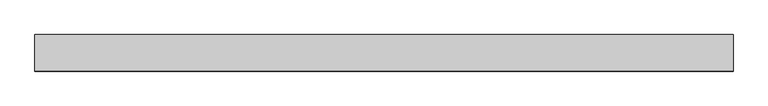
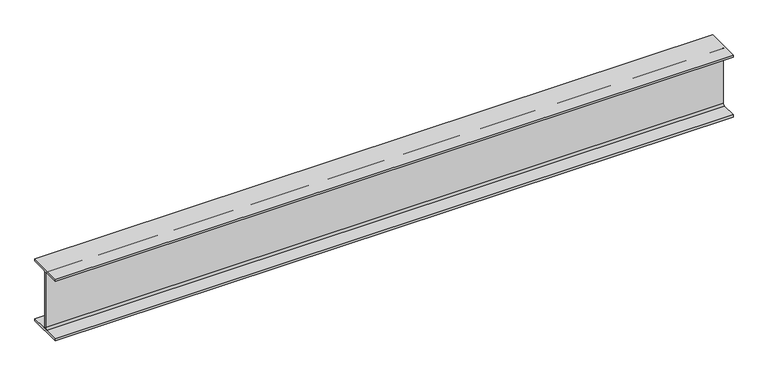
"""IFC4 building model written with IfcOpenShell, lengths in millimetres: beam geometry, Old_Steel Beam_H-KSD3502 : H_SB_ASB_H-250×125x6x9."""

from ifc_helpers import new_model, si_unit, point, frame, frame_2d, origin, place, context, project, spatial, polyline, circle_curve, trimmed, segment, composite_curve, outline, extrude, source, transform, mapped, element, save


def beam_1b59f9ff(model_context):
    return source(origin(), model_context, "Body", "SweptSolid", [
        extrude(outline(composite_curve([segment(polyline([(82.5, -141.5), (82.5, -151.7), (-82.5, -151.7), (-82.5, -141.5), (-11.9, -141.5)]), True, "CONTINUOUS"), segment(trimmed(circle_curve(frame_2d((-11.9, -132.6)), 8.9), [point((-11.9, -141.5))], [point((-3.0, -132.6))], True, "CARTESIAN"), True, "CONTINUOUS"), segment(polyline([(-3.0, -132.6), (-3.0, 132.6)]), True, "CONTINUOUS"), segment(trimmed(circle_curve(frame_2d((-11.9, 132.6)), 8.9), [point((-3.0, 132.6))], [point((-11.9, 141.5))], True, "CARTESIAN"), True, "CONTINUOUS"), segment(polyline([(-11.9, 141.5), (-82.5, 141.5), (-82.5, 151.7), (82.5, 151.7), (82.5, 141.5), (11.9, 141.5)]), True, "CONTINUOUS"), segment(trimmed(circle_curve(frame_2d((11.9, 132.6)), 8.9), [point((11.9, 141.5))], [point((3.0, 132.6))], True, "CARTESIAN"), True, "CONTINUOUS"), segment(polyline([(3.0, 132.6), (3.0, -132.6)]), True, "CONTINUOUS"), segment(trimmed(circle_curve(frame_2d((11.9, -132.6)), 8.9), [point((3.0, -132.6))], [point((11.9, -141.5))], True, "CARTESIAN"), True, "CONTINUOUS"), segment(polyline([(11.9, -141.5), (82.5, -141.5)]), True, "CONTINUOUS")], self_intersect=False)), frame((-1494.4889476, 0.0, 0.0), z_axis=(1.0, 0.0, 0.0), x_axis=(0.0, 1.0, 0.0)), (0.0, 0.0, 1.0), 3149.288991),
    ])


if __name__ == "__main__":
    model = new_model("IFC4")
    model_context = context("Model", 3, world=origin())
    ifc_project = project(units=[si_unit("LENGTHUNIT", "METRE", prefix="MILLI")], contexts=[model_context])
    site = spatial("IfcSite", under=ifc_project)
    building = spatial("IfcBuilding", under=site)
    placement = place(None, origin())
    beam_shape = beam_1b59f9ff(model_context)
    element("IfcBeam", 1, ObjectType="Old_Steel Beam_H-KSD3502 : H_SB_ASB_H-250×125x6x9", at=placement, inside=building, context=model_context, shape_type="MappedRepresentation", body=[
        mapped(beam_shape, transform((0.0, 0.0, 0.0), x_axis=(1.0, 0.0, 0.0), y_axis=(0.0, 1.0, 0.0), z_axis=(0.0, 0.0, 1.0))),
    ])
    save(model, "model.ifc")

# Revit data of these elements
# Type "Old_Steel Beam_H-KSD3502 : H_SB_ASB_H-250×125x6x9"
#   Width = 12.5 cm
#   Web Thickness = 0.6 cm
#   Web Fillet = 1.2 cm
#   Warping Constant = 42539.8 cm⁶
#   Torsional Moment of Inertia = 7.8102 cm⁴
#   Torsional Modulus = 1.0 cm³
#   Section Area = 37.66 cm²
#   Plastic Modulus weak axis = 73.1 cm³
#   Plastic Modulus strong axis = 366.0 cm³
#   Perimeter = 0.97 m²/m
#   Nominal Weight = 29.60 kgf/m
#   Moment of Inertia weak axis = 294.00 cm⁴
#   Moment of Inertia strong axis = 4050.00 cm⁴
#   Height = 25.0 cm
#   Flange Thickness = 0.9 cm
#   Elastic Modulus weak axis = 47.0 cm³
#   Elastic Modulus strong axis = 324.0 cm³
#   Centroid Vertical = 12.5 cm
#   Centroid Horizontal = 6.25 cm
#   Length [instance default] = 1.5240 m
#   Structural Material [instance default] = Steel, 45-345
#   Assembly Code = ""
# Element 1 (IfcBeam, "Old_Steel Beam_H-KSD3502 : H_SB_ASB_H-250×125x6x9")
#   Structural Material = none
# Materials
#   "Steel, 45-345": class "Metal", colour RGB 189 187 185, transparency 0, Description = "Steel 345 MPa", Cost = 0
